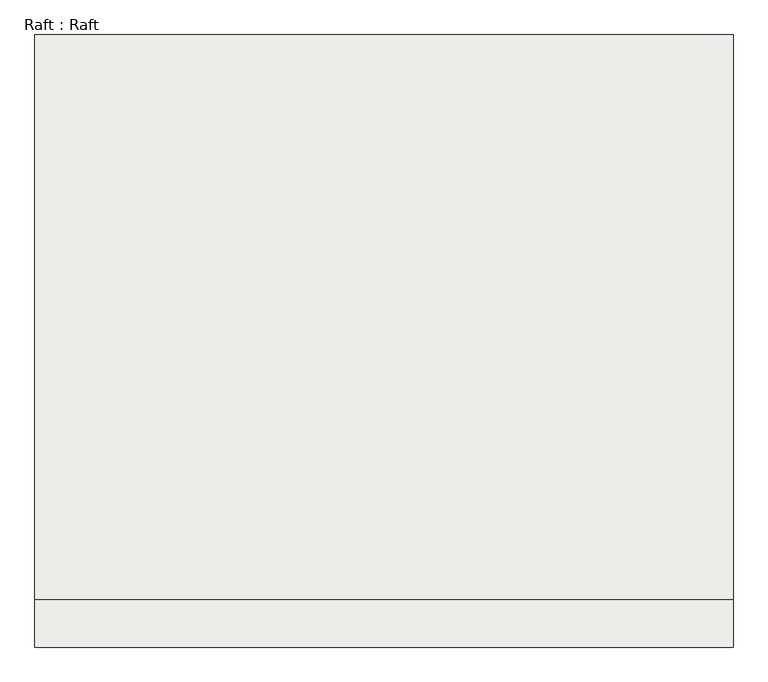
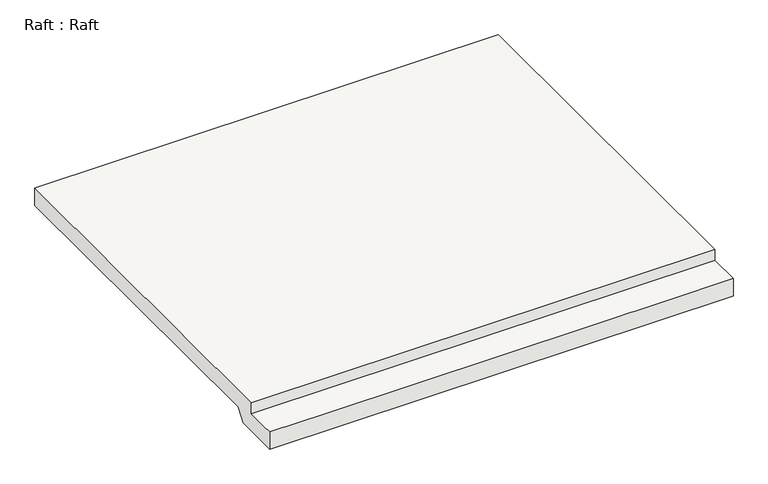
"""IFC4 building model written with IfcOpenShell, lengths in millimetres: slab geometry, Raft : Raft."""

from ifc_helpers import new_model, si_unit, origin, place, context, project, spatial, faceted_brep, source, transform, mapped, element, save


def raft_raft_1b25bfc7(model_context):
    return source(origin(), model_context, "Body", "Brep", [
        faceted_brep([(20200.0, 24700.0, -5320.0), (20200.0, 24300.0, -5320.0), (20200.0, 8199.9985115, -5320.0), (20200.0, 8199.9985115, -5820.0), (20200.0, 6800.0, -5820.0), (20200.0, 6800.0, -6619.9808175), (20200.0, 8809.6095449, -6619.9808175), (20200.0, 9209.5951826, -6120.0), (20200.0, 24700.0, -6120.0), (-200.0, 24700.0, -5320.0), (-200.0, 24700.0, -6120.0), (-200.0, 9209.5951826, -6120.0), (-200.0, 8809.6095449, -6619.9808175), (-200.0, 6800.0, -6619.9808175), (-200.0, 6800.0, -5820.0), (-200.0, 7200.0, -5820.0), (-200.0, 8199.9985115, -5820.0), (-200.0, 8199.9985115, -5320.0), (-200.0, 24300.0, -5320.0), (200.0, 8199.9985115, -5320.0), (19800.0, 8199.9985115, -5320.0), (200.0, 8199.9985115, -5820.0), (19800.0, 8199.9985115, -5820.0), (2300.0, 6800.0, -5820.0), (17700.0, 6800.0, -5820.0), (19800.0, 6800.0, -5820.0)], [[[0, 1, 2, 3, 4, 5, 6, 7, 8]], [[9, 10, 11, 12, 13, 14, 15, 16, 17, 18]], [[2, 1, 0, 9, 18, 17, 19, 20]], [[3, 2, 20, 19, 17, 16, 21, 22]], [[4, 3, 22, 21, 16, 15, 14, 23, 24, 25]], [[5, 4, 25, 24, 23, 14, 13]], [[6, 5, 13, 12]], [[7, 6, 12, 11]], [[8, 7, 11, 10]], [[0, 8, 10, 9]]]),
    ])


if __name__ == "__main__":
    model = new_model("IFC4")
    model_context = context("Model", 3, world=origin())
    ifc_project = project(units=[si_unit("LENGTHUNIT", "METRE", prefix="MILLI")], contexts=[model_context])
    site = spatial("IfcSite", under=ifc_project)
    building = spatial("IfcBuilding", under=site)
    placement = place(None, origin())
    raft_raft_shape = raft_raft_1b25bfc7(model_context)
    element("IfcSlab", 1, ObjectType="Raft : Raft", at=placement, inside=building, context=model_context, shape_type="MappedRepresentation", body=[
        mapped(raft_raft_shape, transform((0.0, 0.0, 0.0), x_axis=(1.0, 0.0, 0.0), y_axis=(0.0, 1.0, 0.0), z_axis=(0.0, 0.0, 1.0))),
    ])
    save(model, "model.ifc")

# Revit data of these elements
# Type "Raft : Raft"
#   Structural Material = Concrete, RC
# Element 1 (IfcSlab, "Raft : Raft")
#   Materials on its faces: "Concrete, RC"
# Materials
#   "Concrete, RC": class "Concrete", colour RGB 116 116 116, transparency 0, Description = "Cast-in-place concrete", Cost = 0
